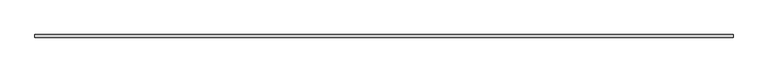
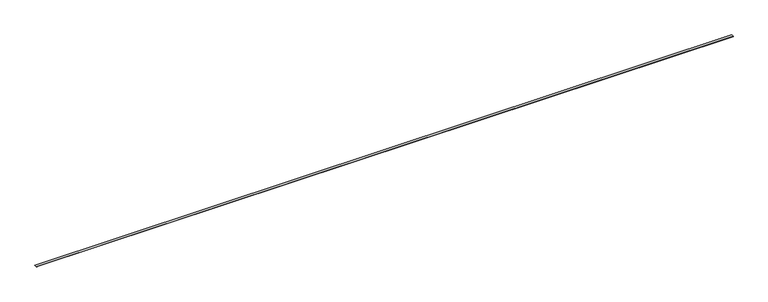
"""IFC4 building model written with IfcOpenShell, lengths in millimetres: proxy geometry, Generic Models 7:Generic Models 1:6:Generic Models 1:6 : Generic Models 7:Generic Models 1:337419:2 : Generic Models 7:Generic Models 1:6:Generic Models 1:6 : Generic Models 7:Generic Models 1:337419:312901."""

from ifc_helpers import new_model, si_unit, frame, origin, place, context, project, spatial, polyline, outline, extrude, source, transform, mapped, element, save


def generic_models_39301db2(model_context):
    return source(origin(), model_context, "Body", "SweptSolid", [
        extrude(outline(polyline([(-578838.7663841, -63.5), (-578873.6913841, -28.575), (-578873.6913841, -12.7), (-578454.5913841, -21.43125), (-578454.5913841, -63.5), (-578838.7663841, -63.5)])), frame((557771.6867239, 0.0, 0.0), z_axis=(1.0, 0.0, 0.0), x_axis=(0.0, 1.0, 0.0)), (0.0, 0.0, 1.0), 109559.725),
    ])


if __name__ == "__main__":
    model = new_model("IFC4")
    model_context = context("Model", 3, world=origin())
    ifc_project = project(units=[si_unit("LENGTHUNIT", "METRE", prefix="MILLI")], contexts=[model_context])
    site = spatial("IfcSite", under=ifc_project)
    building = spatial("IfcBuilding", under=site)
    placement = place(None, origin())
    generic_models_shape = generic_models_39301db2(model_context)
    element("IfcBuildingElementProxy", 1, Name="Generic Models 7:Generic Models 1:6:Generic Models 1:6 : Generic Models 7:Generic Models 1:337419:2 : Generic Models 7:Generic Models 1:6:Generic Models 1:6 : Generic Models 7:Generic Models 1:337419:312901", ObjectType="Generic Models 7:Generic Models 1:6:Generic Models 1:6 : Generic Models 7:Generic Models 1:337419:2 : Generic Models 7:Generic Models 1:6:Generic Models 1:6 : Generic Models 7:Generic Models 1:337419:312901", at=placement, inside=building, context=model_context, shape_type="MappedRepresentation", body=[
        mapped(generic_models_shape, transform((0.0, 0.0, 0.0), x_axis=(1.0, 0.0, 0.0), y_axis=(0.0, 1.0, 0.0), z_axis=(0.0, 0.0, 1.0))),
    ])
    save(model, "model.ifc")

# Revit data of these elements
# Type "Generic Models 7:Generic Models 1:6:Generic Models 1:6 : Generic Models 7:Generic Models 1:337419:2 : Generic Models 7:Generic Models 1:6:Generic Models 1:6 : Generic Models 7:Generic Models 1:337419:312901"
#   NameOverride = "Generic Models 7:Generic Models 1:6:Generic Models 1:6 : Generic Models 7:Generic Models 1:337419:312901"
#   ObjectTypeOverride = "Generic Models 1:6 : Generic Models 7:Generic Models 1:337419"
#   Reference = "Generic Models 1"
#   Tag = "312901"
# Element 1 (IfcBuildingElementProxy, "Generic Models 7:Generic Models 1:6:Generic Models 1:6 : Generic Models 7:Generic Models 1:337419:2 : Generic Models 7:Generic Models 1:6:Generic Models 1:6 : Generic Models 7:Generic Models 1:337419:312901")
#   Materials on its faces: "CONCRETE SLAB - SEE STRUCT DWGS."
# Materials
#   "CONCRETE SLAB - SEE STRUCT DWGS.": class "Concrete", colour RGB 115 116 108, transparency 0, Description = "Lightweight concrete", Cost = 0
